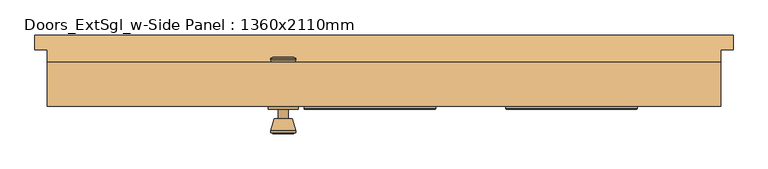
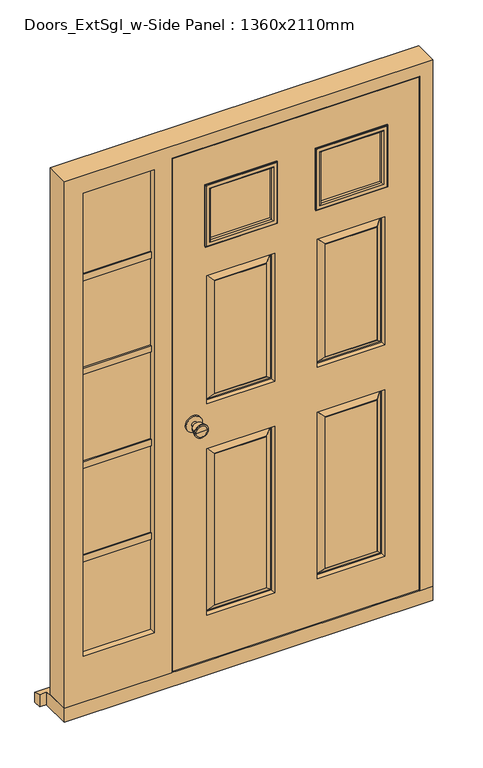
"""IFC4 building model written with IfcOpenShell, lengths in millimetres: door geometry, Doors_ExtSgl_w-Side Panel : 1360x2110mm."""

from ifc_helpers import new_model, si_unit, point, frame, frame_2d, origin, place, context, project, spatial, polyline, circle_curve, ellipse_curve, trimmed, segment, composite_curve, outline, extrude, faceted_brep, source, transform, mapped, element, save
from ifc_brep_helpers import plane_surface, cylinder_surface, revolved_surface, advanced_brep


def doors_extsgl_w_side_panel_1360x2110mm_f8072bf0(model_context):
    return source(origin(), model_context, "Body", "SolidModel", [
        advanced_brep(
        [(-352.5, 25.0, 1000.0), (-342.5, 25.0, 1000.0), (-362.5, 25.0, 1000.0), (-332.0241324, -24.0, 1000.0), (-352.5, -24.0, 1000.0), (-372.9758676, -24.0, 1000.0), (-327.5, -22.1721319, 1000.0), (-377.5, -22.1721319, 1000.0), (-327.5, -18.7084537, 1000.0), (-377.5, -18.7084537, 1000.0), (-333.863764, 6.0, 1000.0), (-371.136236, 6.0, 1000.0), (-342.5, 6.0, 1000.0), (-362.5, 6.0, 1000.0)],
        [
            (0, 1),
            (1, 2, circle_curve(frame((-352.5, 25.0, 1000.0), z_axis=(0.0, 1.0, 0.0), x_axis=(-1.0, 0.0, 0.0)), 10.0)),
            (2, 0),
            (2, 1, circle_curve(frame((-352.5, 25.0, 1000.0), z_axis=(0.0, 1.0, 0.0), x_axis=(-1.0, 0.0, 0.0)), 10.0)),
            (3, 4),
            (4, 5),
            (5, 3, circle_curve(frame((-352.5, -24.0, 1000.0), z_axis=(0.0, -1.0, 0.0), x_axis=(-1.0, 0.0, 0.0)), 20.4758676)),
            (3, 5, circle_curve(frame((-352.5, -24.0, 1000.0), z_axis=(0.0, -1.0, 0.0), x_axis=(-1.0, 0.0, 0.0)), 20.4758676)),
            (6, 3),
            (5, 7),
            (7, 6, circle_curve(frame((-352.5, -22.1721319, 1000.0), z_axis=(0.0, -1.0, 0.0), x_axis=(-1.0, 0.0, 0.0)), 25.0)),
            (6, 7, circle_curve(frame((-352.5, -22.1721319, 1000.0), z_axis=(0.0, -1.0, 0.0), x_axis=(-1.0, 0.0, 0.0)), 25.0)),
            (8, 6),
            (7, 9),
            (9, 8, circle_curve(frame((-352.5, -18.7084537, 1000.0), z_axis=(0.0, -1.0, 0.0), x_axis=(-1.0, 0.0, 0.0)), 25.0)),
            (8, 9, circle_curve(frame((-352.5, -18.7084537, 1000.0), z_axis=(0.0, -1.0, 0.0), x_axis=(-1.0, 0.0, 0.0)), 25.0)),
            (10, 8),
            (9, 11),
            (11, 10, circle_curve(frame((-352.5, 6.0, 1000.0), z_axis=(0.0, -1.0, 0.0), x_axis=(-1.0, 0.0, 0.0)), 18.636236)),
            (10, 11, circle_curve(frame((-352.5, 6.0, 1000.0), z_axis=(0.0, -1.0, 0.0), x_axis=(-1.0, 0.0, 0.0)), 18.636236)),
            (12, 10),
            (11, 13),
            (13, 12, circle_curve(frame((-352.5, 6.0, 1000.0), z_axis=(0.0, -1.0, 0.0), x_axis=(-1.0, 0.0, 0.0)), 10.0)),
            (12, 13, circle_curve(frame((-352.5, 6.0, 1000.0), z_axis=(0.0, -1.0, 0.0), x_axis=(-1.0, 0.0, 0.0)), 10.0)),
            (1, 12),
            (13, 2),
        ],
        [
            plane_surface(frame((-352.5, 25.0, 1000.0), z_axis=(0.0, 1.0, 0.0), x_axis=(-1.0, 0.0, 0.0))),
            plane_surface(frame((-352.5, -24.0, 1000.0), z_axis=(0.0, -1.0, 0.0), x_axis=(-1.0, 0.0, 0.0))),
            revolved_surface(polyline([(-372.9758676, -24.0, 1000.0), (-377.5, -22.1721319, 1000.0)]), (-352.5, 25.0, 1000.0), (0.0, 1.0, 0.0)),
            cylinder_surface(frame((-352.5, 25.0, 1000.0), z_axis=(0.0, 1.0, 0.0), x_axis=(-1.0, 0.0, 0.0)), 25.0),
            revolved_surface(polyline([(-377.5, -18.7084537, 1000.0), (-371.136236, 6.0, 1000.0)]), (-352.5, 25.0, 1000.0), (0.0, 1.0, 0.0)),
            plane_surface(frame((-352.5, 6.0, 1000.0), z_axis=(0.0, 1.0, 0.0), x_axis=(-1.0, 0.0, 0.0))),
            cylinder_surface(frame((-352.5, 25.0, 1000.0), z_axis=(0.0, 1.0, 0.0), x_axis=(-1.0, 0.0, 0.0)), 10.0),
        ],
        [
            (0, [[1, 2, 3]]),
            (0, [[-3, 4, -1]]),
            (1, [[5, 6, 7]]),
            (1, [[-6, -5, 8]]),
            (2, [[9, -7, 10, 11]]),
            (2, [[-10, -8, -9, 12]]),
            (3, [[13, -11, 14, 15]]),
            (3, [[-14, -12, -13, 16]]),
            (4, [[17, -15, 18, 19]]),
            (4, [[-18, -16, -17, 20]]),
            (5, [[21, -19, 22, 23]]),
            (5, [[-22, -20, -21, 24]]),
            (6, [[25, -23, 26, -2]]),
            (6, [[-26, -24, -25, -4]]),
        ],
    ),
        extrude(outline(composite_curve([segment(trimmed(circle_curve(frame_2d((1000.0, -352.5)), 30.0), [point((1000.0, -382.5))], [point((1000.0, -322.5))], False, "CARTESIAN"), True, "CONTINUOUS"), segment(trimmed(circle_curve(frame_2d((1000.0, -352.5)), 30.0), [point((1000.0, -322.5))], [point((1000.0, -382.5))], False, "CARTESIAN"), True, "CONTINUOUS")], self_intersect=False)), frame((0.0, 25.0, 0.0), z_axis=(0.0, 1.0, 0.0), x_axis=(0.0, 0.0, 1.0)), (0.0, 0.0, 1.0), 6.0),
        advanced_brep(
        [(-352.5, 81.0, 1000.0), (-362.5, 81.0, 1000.0), (-342.5, 81.0, 1000.0), (-332.0241324, 130.0, 1000.0), (-372.9758676, 130.0, 1000.0), (-352.5, 130.0, 1000.0), (-327.5, 128.1721319, 1000.0), (-377.5, 128.1721319, 1000.0), (-327.5, 124.7084537, 1000.0), (-377.5, 124.7084537, 1000.0), (-333.863764, 100.0, 1000.0), (-371.136236, 100.0, 1000.0), (-342.5, 100.0, 1000.0), (-362.5, 100.0, 1000.0)],
        [
            (0, 1),
            (1, 2, circle_curve(frame((-352.5, 81.0, 1000.0), z_axis=(0.0, -1.0, 0.0), x_axis=(-1.0, 0.0, 0.0)), 10.0)),
            (2, 0),
            (2, 1, circle_curve(frame((-352.5, 81.0, 1000.0), z_axis=(0.0, -1.0, 0.0), x_axis=(-1.0, 0.0, 0.0)), 10.0)),
            (3, 4, circle_curve(frame((-352.5, 130.0, 1000.0), z_axis=(0.0, 1.0, 0.0), x_axis=(-1.0, 0.0, 0.0)), 20.4758676)),
            (4, 5),
            (5, 3),
            (4, 3, circle_curve(frame((-352.5, 130.0, 1000.0), z_axis=(0.0, 1.0, 0.0), x_axis=(-1.0, 0.0, 0.0)), 20.4758676)),
            (6, 7, circle_curve(frame((-352.5, 128.1721319, 1000.0), z_axis=(0.0, 1.0, 0.0), x_axis=(-1.0, 0.0, 0.0)), 25.0)),
            (7, 4),
            (3, 6),
            (7, 6, circle_curve(frame((-352.5, 128.1721319, 1000.0), z_axis=(0.0, 1.0, 0.0), x_axis=(-1.0, 0.0, 0.0)), 25.0)),
            (8, 9, circle_curve(frame((-352.5, 124.7084537, 1000.0), z_axis=(0.0, 1.0, 0.0), x_axis=(-1.0, 0.0, 0.0)), 25.0)),
            (9, 7),
            (6, 8),
            (9, 8, circle_curve(frame((-352.5, 124.7084537, 1000.0), z_axis=(0.0, 1.0, 0.0), x_axis=(-1.0, 0.0, 0.0)), 25.0)),
            (10, 11, circle_curve(frame((-352.5, 100.0, 1000.0), z_axis=(0.0, 1.0, 0.0), x_axis=(-1.0, 0.0, 0.0)), 18.636236)),
            (11, 9),
            (8, 10),
            (11, 10, circle_curve(frame((-352.5, 100.0, 1000.0), z_axis=(0.0, 1.0, 0.0), x_axis=(-1.0, 0.0, 0.0)), 18.636236)),
            (12, 13, circle_curve(frame((-352.5, 100.0, 1000.0), z_axis=(0.0, 1.0, 0.0), x_axis=(-1.0, 0.0, 0.0)), 10.0)),
            (13, 11),
            (10, 12),
            (13, 12, circle_curve(frame((-352.5, 100.0, 1000.0), z_axis=(0.0, 1.0, 0.0), x_axis=(-1.0, 0.0, 0.0)), 10.0)),
            (1, 13),
            (12, 2),
        ],
        [
            plane_surface(frame((-352.5, 81.0, 1000.0), z_axis=(0.0, -1.0, 0.0), x_axis=(-1.0, 0.0, 0.0))),
            plane_surface(frame((-352.5, 130.0, 1000.0), z_axis=(0.0, 1.0, 0.0), x_axis=(-1.0, 0.0, 0.0))),
            revolved_surface(polyline([(-372.9758676, 130.0, 1000.0), (-377.5, 128.1721319, 1000.0)]), (-352.5, 81.0, 1000.0), (0.0, -1.0, 0.0)),
            cylinder_surface(frame((-352.5, 81.0, 1000.0), z_axis=(0.0, -1.0, 0.0), x_axis=(-1.0, 0.0, 0.0)), 25.0),
            revolved_surface(polyline([(-377.5, 124.7084537, 1000.0), (-371.136236, 100.0, 1000.0)]), (-352.5, 81.0, 1000.0), (0.0, -1.0, 0.0)),
            plane_surface(frame((-352.5, 100.0, 1000.0), z_axis=(0.0, -1.0, 0.0), x_axis=(-1.0, 0.0, 0.0))),
            cylinder_surface(frame((-352.5, 81.0, 1000.0), z_axis=(0.0, -1.0, 0.0), x_axis=(-1.0, 0.0, 0.0)), 10.0),
        ],
        [
            (0, [[1, 2, 3]]),
            (0, [[-3, 4, -1]]),
            (1, [[5, 6, 7]]),
            (1, [[8, -7, -6]]),
            (2, [[9, 10, -5, 11]]),
            (2, [[12, -11, -8, -10]]),
            (3, [[13, 14, -9, 15]]),
            (3, [[16, -15, -12, -14]]),
            (4, [[17, 18, -13, 19]]),
            (4, [[20, -19, -16, -18]]),
            (5, [[21, 22, -17, 23]]),
            (5, [[24, -23, -20, -22]]),
            (6, [[-2, 25, -21, 26]]),
            (6, [[-4, -26, -24, -25]]),
        ],
    ),
        extrude(outline(composite_curve([segment(trimmed(circle_curve(frame_2d((1000.0, -352.5)), 30.0), [point((1000.0, -382.5))], [point((1000.0, -322.5))], False, "CARTESIAN"), True, "CONTINUOUS"), segment(trimmed(circle_curve(frame_2d((1000.0, -352.5)), 30.0), [point((1000.0, -322.5))], [point((1000.0, -382.5))], False, "CARTESIAN"), True, "CONTINUOUS")], self_intersect=False)), frame((0.0, 75.0, 0.0), z_axis=(0.0, 1.0, 0.0), x_axis=(0.0, 0.0, 1.0)), (0.0, 0.0, 1.0), 6.0),
        faceted_brep([(460.5, 120.0, 54.5), (531.0, 120.0, 54.5), (531.0, 31.0, 54.5), (482.5, 31.0, 54.5), (482.5, 78.0, 54.5), (460.5, 78.0, 54.5), (460.5, 120.0, 2039.5), (-410.5, 120.0, 2039.5), (-410.5, 120.0, 54.5), (-829.0, 120.0, 54.5), (-829.0, 120.0, 2110.0), (531.0, 120.0, 2110.0), (-496.5, 120.0, 2039.5), (-758.5, 120.0, 2039.5), (-758.5, 120.0, 233.5), (-496.5, 120.0, 233.5), (531.0, 31.0, 2110.0), (-829.0, 31.0, 2110.0), (-829.0, 31.0, 54.5), (-432.5, 31.0, 54.5), (-432.5, 31.0, 2061.5), (482.5, 31.0, 2061.5), (-496.5, 31.0, 233.5), (-758.5, 31.0, 233.5), (-758.5, 31.0, 2039.5), (-496.5, 31.0, 2039.5), (482.5, 78.0, 2061.5), (-432.5, 78.0, 2061.5), (-432.5, 78.0, 54.5), (-410.5, 78.0, 54.5), (-410.5, 78.0, 2039.5), (460.5, 78.0, 2039.5), (-474.5, 78.0, 2061.5), (-780.5, 78.0, 2061.5), (-780.5, 78.0, 218.5), (-474.5, 78.0, 218.5), (-758.5, 78.0, 2039.5), (-496.5, 78.0, 2039.5), (-496.5, 78.0, 233.5), (-758.5, 78.0, 233.5), (-496.5, 54.0, 233.5), (-758.5, 54.0, 233.5), (-758.5, 54.0, 2039.5), (-496.5, 54.0, 2039.5), (-780.5, 54.0, 2061.5), (-780.5, 54.0, 218.5), (-474.5, 54.0, 218.5), (-474.5, 54.0, 2061.5)], [[[0, 1, 2, 3, 4, 5]], [[1, 0, 6, 7, 8, 9, 10, 11], [12, 13, 14, 15]], [[2, 1, 11, 16]], [[3, 2, 16, 17, 18, 19, 20, 21], [22, 23, 24, 25]], [[4, 3, 21, 26]], [[5, 4, 26, 27, 28, 29, 30, 31]], [[32, 33, 34, 35], [36, 37, 38, 39]], [[0, 5, 31, 6]], [[29, 8, 7, 30]], [[18, 9, 8, 29, 28, 19]], [[10, 9, 18, 17]], [[13, 36, 39, 14]], [[39, 38, 15, 14]], [[37, 12, 15, 38]], [[23, 22, 40, 41]], [[24, 23, 41, 42]], [[22, 25, 43, 40]], [[19, 28, 27, 20]], [[44, 45, 34, 33]], [[45, 46, 35, 34]], [[46, 47, 32, 35]], [[46, 45, 44, 47], [41, 40, 43, 42]], [[11, 10, 17, 16]], [[26, 21, 20, 27]], [[33, 32, 47, 44]], [[6, 31, 30, 7]], [[36, 13, 12, 37]], [[25, 24, 42, 43]]]),
        extrude(outline(polyline([(354.5, 41.0), (104.5, 41.0), (104.5, 65.0), (354.5, 65.0), (354.5, 41.0)])), frame((0.0, 0.0, 1683.5), z_axis=(0.0, 0.0, 1.0), x_axis=(1.0, 0.0, 0.0)), (0.0, 0.0, 1.0), 225.0),
        extrude(outline(polyline([(-52.5, 41.0), (-302.5, 41.0), (-302.5, 65.0), (-52.5, 65.0), (-52.5, 41.0)])), frame((0.0, 0.0, 1683.5), z_axis=(0.0, 0.0, 1.0), x_axis=(1.0, 0.0, 0.0)), (0.0, 0.0, 1.0), 225.0),
        faceted_brep([(556.0, 175.0, 0.0), (556.0, 175.0, 38.5947221), (556.0, 145.0, 47.2703282), (556.0, 145.0, 0.0), (-854.0, 175.0, 38.5947221), (-854.0, 175.0, 0.0), (-854.0, 145.0, 0.0), (-854.0, 145.0, 47.2703282), (531.0, 145.0, 0.0), (531.0, 31.0, 0.0), (-829.0, 31.0, 0.0), (-829.0, 145.0, 0.0), (-829.0, 145.0, 47.2703282), (-829.0, 120.0, 54.5), (531.0, 120.0, 54.5), (531.0, 145.0, 47.2703282), (-829.0, 31.0, 54.5), (531.0, 31.0, 54.5)], [[[0, 1, 2, 3]], [[4, 5, 6, 7]], [[5, 0, 3, 8, 9, 10, 11, 6]], [[1, 0, 5, 4]], [[1, 4, 7, 12, 13, 14, 15, 2]], [[13, 16, 17, 14]], [[16, 10, 9, 17]], [[12, 11, 10, 16, 13]], [[11, 12, 7, 6]], [[8, 15, 14, 17, 9]], [[15, 8, 3, 2]]]),
        faceted_brep([(479.5, 31.0, 58.5), (479.5, 31.0, 2058.5), (-427.5, 31.0, 2058.5), (-427.5, 31.0, 58.5), (104.5, 31.0, 1683.5), (104.5, 31.0, 1908.5), (354.5, 31.0, 1908.5), (354.5, 31.0, 1683.5), (-302.5, 31.0, 1683.5), (-302.5, 31.0, 1908.5), (-52.5, 31.0, 1908.5), (-52.5, 31.0, 1683.5), (-52.5, 31.0, 883.5), (-52.5, 31.0, 233.5), (-302.5, 31.0, 233.5), (-302.5, 31.0, 883.5), (354.5, 31.0, 883.5), (354.5, 31.0, 233.5), (104.5, 31.0, 233.5), (104.5, 31.0, 883.5), (-52.5, 31.0, 1558.5), (-52.5, 31.0, 1058.5), (-302.5, 31.0, 1058.5), (-302.5, 31.0, 1558.5), (354.5, 31.0, 1558.5), (354.5, 31.0, 1058.5), (104.5, 31.0, 1058.5), (104.5, 31.0, 1558.5), (-82.5, 31.0, 263.5), (-82.5, 31.0, 853.5), (-272.5, 31.0, 853.5), (-272.5, 31.0, 263.5), (324.5, 31.0, 263.5), (324.5, 31.0, 853.5), (134.5, 31.0, 853.5), (134.5, 31.0, 263.5), (-82.5, 31.0, 1088.5), (-82.5, 31.0, 1528.5), (-272.5, 31.0, 1528.5), (-272.5, 31.0, 1088.5), (324.5, 31.0, 1088.5), (324.5, 31.0, 1528.5), (134.5, 31.0, 1528.5), (134.5, 31.0, 1088.5), (479.5, 75.0, 58.5), (-427.5, 75.0, 58.5), (-427.5, 75.0, 2058.5), (479.5, 75.0, 2058.5), (104.5, 75.0, 1683.5), (354.5, 75.0, 1683.5), (354.5, 75.0, 1908.5), (104.5, 75.0, 1908.5), (-302.5, 75.0, 1683.5), (-52.5, 75.0, 1683.5), (-52.5, 75.0, 1908.5), (-302.5, 75.0, 1908.5), (104.5, 75.0, 883.5), (104.5, 75.0, 233.5), (354.5, 75.0, 233.5), (354.5, 75.0, 883.5), (-302.5, 75.0, 883.5), (-302.5, 75.0, 233.5), (-52.5, 75.0, 233.5), (-52.5, 75.0, 883.5), (104.5, 75.0, 1558.5), (104.5, 75.0, 1058.5), (354.5, 75.0, 1058.5), (354.5, 75.0, 1558.5), (-302.5, 75.0, 1558.5), (-302.5, 75.0, 1058.5), (-52.5, 75.0, 1058.5), (-52.5, 75.0, 1558.5), (134.5, 75.0, 263.5), (134.5, 75.0, 853.5), (324.5, 75.0, 853.5), (324.5, 75.0, 263.5), (-272.5, 75.0, 263.5), (-272.5, 75.0, 853.5), (-82.5, 75.0, 853.5), (-82.5, 75.0, 263.5), (134.5, 75.0, 1088.5), (134.5, 75.0, 1528.5), (324.5, 75.0, 1528.5), (324.5, 75.0, 1088.5), (-272.5, 75.0, 1088.5), (-272.5, 75.0, 1528.5), (-82.5, 75.0, 1528.5), (-82.5, 75.0, 1088.5), (107.5, 60.0, 880.5), (107.5, 60.0, 236.5), (132.5, 74.0, 855.5), (132.5, 74.0, 261.5), (112.5, 60.0, 241.5), (112.5, 60.0, 875.5), (134.5, 74.0, 263.5), (134.5, 74.0, 853.5), (351.5, 60.0, 236.5), (326.5, 74.0, 261.5), (346.5, 60.0, 241.5), (324.5, 74.0, 263.5), (351.5, 60.0, 880.5), (326.5, 74.0, 855.5), (346.5, 60.0, 875.5), (324.5, 74.0, 853.5), (-299.5, 60.0, 880.5), (-299.5, 60.0, 236.5), (-274.5, 74.0, 855.5), (-274.5, 74.0, 261.5), (-294.5, 60.0, 241.5), (-294.5, 60.0, 875.5), (-272.5, 74.0, 263.5), (-272.5, 74.0, 853.5), (-55.5, 60.0, 236.5), (-80.5, 74.0, 261.5), (-60.5, 60.0, 241.5), (-82.5, 74.0, 263.5), (-55.5, 60.0, 880.5), (-80.5, 74.0, 855.5), (-60.5, 60.0, 875.5), (-82.5, 74.0, 853.5), (-82.5, 32.0, 263.5), (-82.5, 32.0, 853.5), (-60.5, 46.0, 241.5), (-60.5, 46.0, 875.5), (-80.5, 32.0, 855.5), (-80.5, 32.0, 261.5), (-55.5, 46.0, 880.5), (-55.5, 46.0, 236.5), (-272.5, 32.0, 853.5), (-294.5, 46.0, 875.5), (-274.5, 32.0, 855.5), (-299.5, 46.0, 880.5), (-272.5, 32.0, 263.5), (-294.5, 46.0, 241.5), (-274.5, 32.0, 261.5), (-299.5, 46.0, 236.5), (351.5, 46.0, 880.5), (351.5, 46.0, 236.5), (326.5, 32.0, 855.5), (326.5, 32.0, 261.5), (346.5, 46.0, 241.5), (346.5, 46.0, 875.5), (324.5, 32.0, 263.5), (324.5, 32.0, 853.5), (107.5, 46.0, 236.5), (132.5, 32.0, 261.5), (112.5, 46.0, 241.5), (134.5, 32.0, 263.5), (107.5, 46.0, 880.5), (132.5, 32.0, 855.5), (112.5, 46.0, 875.5), (134.5, 32.0, 853.5), (134.5, 74.0, 1088.5), (134.5, 74.0, 1528.5), (112.5, 60.0, 1066.5), (112.5, 60.0, 1550.5), (132.5, 74.0, 1530.5), (132.5, 74.0, 1086.5), (107.5, 60.0, 1555.5), (107.5, 60.0, 1061.5), (324.5, 74.0, 1528.5), (346.5, 60.0, 1550.5), (326.5, 74.0, 1530.5), (351.5, 60.0, 1555.5), (324.5, 74.0, 1088.5), (346.5, 60.0, 1066.5), (326.5, 74.0, 1086.5), (351.5, 60.0, 1061.5), (-272.5, 74.0, 1088.5), (-272.5, 74.0, 1528.5), (-294.5, 60.0, 1066.5), (-294.5, 60.0, 1550.5), (-274.5, 74.0, 1530.5), (-274.5, 74.0, 1086.5), (-299.5, 60.0, 1555.5), (-299.5, 60.0, 1061.5), (-82.5, 74.0, 1528.5), (-60.5, 60.0, 1550.5), (-80.5, 74.0, 1530.5), (-55.5, 60.0, 1555.5), (-82.5, 74.0, 1088.5), (-60.5, 60.0, 1066.5), (-80.5, 74.0, 1086.5), (-55.5, 60.0, 1061.5), (-82.5, 32.0, 1088.5), (-82.5, 32.0, 1528.5), (-60.5, 46.0, 1066.5), (-60.5, 46.0, 1550.5), (-80.5, 32.0, 1530.5), (-80.5, 32.0, 1086.5), (-55.5, 46.0, 1555.5), (-55.5, 46.0, 1061.5), (-272.5, 32.0, 1528.5), (-294.5, 46.0, 1550.5), (-274.5, 32.0, 1530.5), (-299.5, 46.0, 1555.5), (-272.5, 32.0, 1088.5), (-294.5, 46.0, 1066.5), (-274.5, 32.0, 1086.5), (-299.5, 46.0, 1061.5), (351.5, 46.0, 1555.5), (351.5, 46.0, 1061.5), (326.5, 32.0, 1530.5), (326.5, 32.0, 1086.5), (346.5, 46.0, 1066.5), (346.5, 46.0, 1550.5), (324.5, 32.0, 1088.5), (324.5, 32.0, 1528.5), (107.5, 46.0, 1061.5), (132.5, 32.0, 1086.5), (112.5, 46.0, 1066.5), (134.5, 32.0, 1088.5), (107.5, 46.0, 1555.5), (132.5, 32.0, 1530.5), (112.5, 46.0, 1550.5), (134.5, 32.0, 1528.5)], [[[0, 1, 2, 3], [4, 5, 6, 7], [8, 9, 10, 11], [12, 13, 14, 15], [16, 17, 18, 19], [20, 21, 22, 23], [24, 25, 26, 27]], [[28, 29, 30, 31]], [[32, 33, 34, 35]], [[36, 37, 38, 39]], [[40, 41, 42, 43]], [[44, 45, 46, 47], [48, 49, 50, 51], [52, 53, 54, 55], [56, 57, 58, 59], [60, 61, 62, 63], [64, 65, 66, 67], [68, 69, 70, 71]], [[72, 73, 74, 75]], [[76, 77, 78, 79]], [[80, 81, 82, 83]], [[84, 85, 86, 87]], [[1, 0, 44, 47]], [[2, 1, 47, 46]], [[3, 2, 46, 45]], [[0, 3, 45, 44]], [[5, 4, 48, 51]], [[6, 5, 51, 50]], [[7, 6, 50, 49]], [[4, 7, 49, 48]], [[9, 8, 52, 55]], [[10, 9, 55, 54]], [[11, 10, 54, 53]], [[8, 11, 53, 52]], [[88, 89, 57, 56]], [[90, 91, 92, 93]], [[72, 94, 95, 73]], [[57, 89, 96, 58]], [[92, 91, 97, 98]], [[94, 72, 75, 99]], [[58, 96, 100, 59]], [[98, 97, 101, 102]], [[99, 75, 74, 103]], [[88, 56, 59, 100]], [[89, 88, 100, 96], [93, 92, 98, 102]], [[90, 93, 102, 101]], [[91, 90, 101, 97], [95, 94, 99, 103]], [[73, 95, 103, 74]], [[104, 105, 61, 60]], [[106, 107, 108, 109]], [[76, 110, 111, 77]], [[61, 105, 112, 62]], [[108, 107, 113, 114]], [[110, 76, 79, 115]], [[62, 112, 116, 63]], [[114, 113, 117, 118]], [[115, 79, 78, 119]], [[104, 60, 63, 116]], [[105, 104, 116, 112], [109, 108, 114, 118]], [[106, 109, 118, 117]], [[107, 106, 117, 113], [111, 110, 115, 119]], [[77, 111, 119, 78]], [[120, 121, 29, 28]], [[122, 123, 124, 125]], [[12, 126, 127, 13]], [[29, 121, 128, 30]], [[124, 123, 129, 130]], [[126, 12, 15, 131]], [[30, 128, 132, 31]], [[130, 129, 133, 134]], [[131, 15, 14, 135]], [[120, 28, 31, 132]], [[125, 124, 130, 134], [121, 120, 132, 128]], [[122, 125, 134, 133]], [[127, 126, 131, 135], [123, 122, 133, 129]], [[13, 127, 135, 14]], [[136, 137, 17, 16]], [[138, 139, 140, 141]], [[32, 142, 143, 33]], [[17, 137, 144, 18]], [[140, 139, 145, 146]], [[142, 32, 35, 147]], [[18, 144, 148, 19]], [[146, 145, 149, 150]], [[147, 35, 34, 151]], [[136, 16, 19, 148]], [[137, 136, 148, 144], [141, 140, 146, 150]], [[138, 141, 150, 149]], [[139, 138, 149, 145], [143, 142, 147, 151]], [[33, 143, 151, 34]], [[152, 153, 81, 80]], [[154, 155, 156, 157]], [[64, 158, 159, 65]], [[81, 153, 160, 82]], [[156, 155, 161, 162]], [[158, 64, 67, 163]], [[82, 160, 164, 83]], [[162, 161, 165, 166]], [[163, 67, 66, 167]], [[152, 80, 83, 164]], [[157, 156, 162, 166], [153, 152, 164, 160]], [[154, 157, 166, 165]], [[159, 158, 163, 167], [155, 154, 165, 161]], [[65, 159, 167, 66]], [[168, 169, 85, 84]], [[170, 171, 172, 173]], [[68, 174, 175, 69]], [[85, 169, 176, 86]], [[172, 171, 177, 178]], [[174, 68, 71, 179]], [[86, 176, 180, 87]], [[178, 177, 181, 182]], [[179, 71, 70, 183]], [[168, 84, 87, 180]], [[173, 172, 178, 182], [169, 168, 180, 176]], [[170, 173, 182, 181]], [[175, 174, 179, 183], [171, 170, 181, 177]], [[69, 175, 183, 70]], [[184, 185, 37, 36]], [[186, 187, 188, 189]], [[20, 190, 191, 21]], [[37, 185, 192, 38]], [[188, 187, 193, 194]], [[190, 20, 23, 195]], [[38, 192, 196, 39]], [[194, 193, 197, 198]], [[195, 23, 22, 199]], [[184, 36, 39, 196]], [[189, 188, 194, 198], [185, 184, 196, 192]], [[186, 189, 198, 197]], [[191, 190, 195, 199], [187, 186, 197, 193]], [[21, 191, 199, 22]], [[200, 201, 25, 24]], [[202, 203, 204, 205]], [[40, 206, 207, 41]], [[25, 201, 208, 26]], [[204, 203, 209, 210]], [[206, 40, 43, 211]], [[26, 208, 212, 27]], [[210, 209, 213, 214]], [[211, 43, 42, 215]], [[200, 24, 27, 212]], [[201, 200, 212, 208], [205, 204, 210, 214]], [[202, 205, 214, 213]], [[203, 202, 213, 209], [207, 206, 211, 215]], [[41, 207, 215, 42]]]),
        advanced_brep(
        [(362.5, 27.0, 1675.5), (362.5, 31.0, 1675.5), (362.5, 31.0, 1916.5), (362.5, 27.0, 1916.5), (360.5, 25.0, 1677.5), (360.5, 25.0, 1914.5), (342.5, 30.0, 1695.5), (347.5, 25.0, 1690.5), (347.5, 25.0, 1901.5), (342.5, 30.0, 1896.5), (342.5, 41.0, 1695.5), (342.5, 41.0, 1896.5), (354.5, 31.0, 1683.5), (354.5, 41.0, 1683.5), (354.5, 41.0, 1908.5), (354.5, 31.0, 1908.5), (96.5, 31.0, 1916.5), (96.5, 27.0, 1916.5), (98.5, 25.0, 1914.5), (111.5, 25.0, 1901.5), (116.5, 30.0, 1896.5), (116.5, 41.0, 1896.5), (104.5, 41.0, 1908.5), (104.5, 31.0, 1908.5), (96.5, 31.0, 1675.5), (96.5, 27.0, 1675.5), (98.5, 25.0, 1677.5), (111.5, 25.0, 1690.5), (116.5, 30.0, 1695.5), (116.5, 41.0, 1695.5), (104.5, 41.0, 1683.5), (104.5, 31.0, 1683.5)],
        [
            (0, 1),
            (1, 2),
            (2, 3),
            (3, 0),
            (4, 0, ellipse_curve(frame((360.5, 27.0, 1677.5), z_axis=(0.7071067811865475, 0.0, 0.7071067811865475), x_axis=(0.7071067811865474, 0.0, -0.7071067811865476)), 2.8284271, 2.0)),
            (3, 5, ellipse_curve(frame((360.5, 27.0, 1914.5), z_axis=(0.7071067811865475, 0.0, -0.7071067811865475), x_axis=(-0.7071067811865474, 0.0, -0.7071067811865476)), 2.8284271, 2.0)),
            (5, 4),
            (6, 7, ellipse_curve(frame((347.5, 30.0, 1690.5), z_axis=(0.7071067811865475, 0.0, 0.7071067811865475), x_axis=(0.7071067811865474, 0.0, -0.7071067811865476)), 7.0710678, 5.0)),
            (7, 8),
            (8, 9, ellipse_curve(frame((347.5, 30.0, 1901.5), z_axis=(0.7071067811865475, 0.0, -0.7071067811865475), x_axis=(-0.7071067811865474, 0.0, -0.7071067811865476)), 7.0710678, 5.0)),
            (9, 6),
            (10, 6),
            (9, 11),
            (11, 10),
            (12, 13),
            (13, 14),
            (14, 15),
            (15, 12),
            (2, 16),
            (16, 17),
            (17, 3),
            (17, 18, ellipse_curve(frame((98.5, 27.0, 1914.5), z_axis=(0.7071067811865475, 0.0, 0.7071067811865475), x_axis=(0.7071067811865476, 0.0, -0.7071067811865474)), 2.8284271, 2.0)),
            (18, 5),
            (8, 19),
            (19, 20, ellipse_curve(frame((111.5, 30.0, 1901.5), z_axis=(0.7071067811865475, 0.0, 0.7071067811865475), x_axis=(0.7071067811865476, 0.0, -0.7071067811865474)), 7.0710678, 5.0)),
            (20, 9),
            (20, 21),
            (21, 11),
            (14, 22),
            (22, 23),
            (23, 15),
            (16, 24),
            (24, 25),
            (25, 17),
            (25, 26, ellipse_curve(frame((98.5, 27.0, 1677.5), z_axis=(-0.7071067811865475, 0.0, 0.7071067811865475), x_axis=(0.7071067811865474, 0.0, 0.7071067811865476)), 2.8284271, 2.0)),
            (26, 18),
            (19, 27),
            (27, 28, ellipse_curve(frame((111.5, 30.0, 1690.5), z_axis=(-0.7071067811865475, 0.0, 0.7071067811865475), x_axis=(0.7071067811865474, 0.0, 0.7071067811865476)), 7.0710678, 5.0)),
            (28, 20),
            (28, 29),
            (29, 21),
            (22, 30),
            (30, 31),
            (31, 23),
            (24, 1),
            (0, 25),
            (4, 26),
            (7, 27),
            (6, 28),
            (10, 29),
            (13, 30),
            (12, 31),
        ],
        [
            plane_surface(frame((362.5, 31.0, 1675.5), z_axis=(1.0, 0.0, 0.0), x_axis=(0.0, 0.0, 1.0))),
            cylinder_surface(frame((360.5, 27.0, 1683.5), z_axis=(0.0, 0.0, -1.0), x_axis=(1.0, 0.0, 0.0)), 2.0),
            cylinder_surface(frame((347.5, 30.0, 1683.5), z_axis=(0.0, 0.0, -1.0), x_axis=(1.0, 0.0, 0.0)), 5.0),
            plane_surface(frame((342.5, 30.0, 1695.5), z_axis=(-1.0, 0.0, 0.0), x_axis=(0.0, 0.0, 1.0))),
            plane_surface(frame((354.5, 41.0, 1683.5), z_axis=(1.0, 0.0, 0.0), x_axis=(0.0, 0.0, 1.0))),
            plane_surface(frame((362.5, 31.0, 1916.5), z_axis=(0.0, 0.0, 1.0), x_axis=(-1.0, 0.0, 0.0))),
            cylinder_surface(frame((354.5, 27.0, 1914.5), z_axis=(1.0, 0.0, 0.0), x_axis=(0.0, 0.0, 1.0)), 2.0),
            cylinder_surface(frame((354.5, 30.0, 1901.5), z_axis=(1.0, 0.0, 0.0), x_axis=(0.0, 0.0, 1.0)), 5.0),
            plane_surface(frame((342.5, 30.0, 1896.5), z_axis=(0.0, 0.0, -1.0), x_axis=(-1.0, 0.0, 0.0))),
            plane_surface(frame((354.5, 41.0, 1908.5), z_axis=(0.0, 0.0, 1.0), x_axis=(-1.0, 0.0, 0.0))),
            plane_surface(frame((96.5, 31.0, 1916.5), z_axis=(-1.0, 0.0, 0.0), x_axis=(0.0, 0.0, -1.0))),
            cylinder_surface(frame((98.5, 27.0, 1908.5), z_axis=(0.0, 0.0, 1.0), x_axis=(-1.0, 0.0, 0.0)), 2.0),
            cylinder_surface(frame((111.5, 30.0, 1908.5), z_axis=(0.0, 0.0, 1.0), x_axis=(-1.0, 0.0, 0.0)), 5.0),
            plane_surface(frame((116.5, 30.0, 1896.5), z_axis=(1.0, 0.0, 0.0), x_axis=(0.0, 0.0, -1.0))),
            plane_surface(frame((104.5, 41.0, 1908.5), z_axis=(-1.0, 0.0, 0.0), x_axis=(0.0, 0.0, -1.0))),
            plane_surface(frame((96.5, 31.0, 1675.5), z_axis=(0.0, 0.0, -1.0), x_axis=(1.0, 0.0, 0.0))),
            cylinder_surface(frame((104.5, 27.0, 1677.5), z_axis=(-1.0, 0.0, 0.0), x_axis=(0.0, 0.0, -1.0)), 2.0),
            plane_surface(frame((98.5, 25.0, 1677.5), z_axis=(0.0, -1.0, 0.0), x_axis=(1.0, 0.0, 0.0))),
            cylinder_surface(frame((104.5, 30.0, 1690.5), z_axis=(-1.0, 0.0, 0.0), x_axis=(0.0, 0.0, -1.0)), 5.0),
            plane_surface(frame((116.5, 30.0, 1695.5), z_axis=(0.0, 0.0, 1.0), x_axis=(1.0, 0.0, 0.0))),
            plane_surface(frame((116.5, 41.0, 1695.5), z_axis=(0.0, 1.0, 0.0), x_axis=(1.0, 0.0, 0.0))),
            plane_surface(frame((104.5, 41.0, 1683.5), z_axis=(0.0, 0.0, -1.0), x_axis=(1.0, 0.0, 0.0))),
            plane_surface(frame((104.5, 31.0, 1683.5), z_axis=(0.0, 1.0, 0.0), x_axis=(1.0, 0.0, 0.0))),
        ],
        [
            (0, [[1, 2, 3, 4]]),
            (1, [[5, -4, 6, 7]]),
            (2, [[8, 9, 10, 11]]),
            (3, [[12, -11, 13, 14]]),
            (4, [[15, 16, 17, 18]]),
            (5, [[-3, 19, 20, 21]]),
            (6, [[-6, -21, 22, 23]]),
            (7, [[-10, 24, 25, 26]]),
            (8, [[-13, -26, 27, 28]]),
            (9, [[-17, 29, 30, 31]]),
            (10, [[-20, 32, 33, 34]]),
            (11, [[-22, -34, 35, 36]]),
            (12, [[-25, 37, 38, 39]]),
            (13, [[-27, -39, 40, 41]]),
            (14, [[-30, 42, 43, 44]]),
            (15, [[-33, 45, -1, 46]]),
            (16, [[-35, -46, -5, 47]]),
            (17, [[-23, -36, -47, -7], [48, -37, -24, -9]]),
            (18, [[-38, -48, -8, 49]]),
            (19, [[-40, -49, -12, 50]]),
            (20, [[51, -42, -29, -16], [-28, -41, -50, -14]]),
            (21, [[-43, -51, -15, 52]]),
            (22, [[-45, -32, -19, -2], [-31, -44, -52, -18]]),
        ],
    ),
        advanced_brep(
        [(-44.5, 27.0, 1675.5), (-44.5, 31.0, 1675.5), (-44.5, 31.0, 1916.5), (-44.5, 27.0, 1916.5), (-46.5, 25.0, 1677.5), (-46.5, 25.0, 1914.5), (-64.5, 30.0, 1695.5), (-59.5, 25.0, 1690.5), (-59.5, 25.0, 1901.5), (-64.5, 30.0, 1896.5), (-64.5, 41.0, 1695.5), (-64.5, 41.0, 1896.5), (-52.5, 31.0, 1683.5), (-52.5, 41.0, 1683.5), (-52.5, 41.0, 1908.5), (-52.5, 31.0, 1908.5), (-310.5, 31.0, 1916.5), (-310.5, 27.0, 1916.5), (-308.5, 25.0, 1914.5), (-295.5, 25.0, 1901.5), (-290.5, 30.0, 1896.5), (-290.5, 41.0, 1896.5), (-302.5, 41.0, 1908.5), (-302.5, 31.0, 1908.5), (-310.5, 31.0, 1675.5), (-310.5, 27.0, 1675.5), (-308.5, 25.0, 1677.5), (-295.5, 25.0, 1690.5), (-290.5, 30.0, 1695.5), (-290.5, 41.0, 1695.5), (-302.5, 41.0, 1683.5), (-302.5, 31.0, 1683.5)],
        [
            (0, 1),
            (1, 2),
            (2, 3),
            (3, 0),
            (4, 0, ellipse_curve(frame((-46.5, 27.0, 1677.5), z_axis=(0.7071067811865475, 0.0, 0.7071067811865475), x_axis=(0.7071067811865474, 0.0, -0.7071067811865476)), 2.8284271, 2.0)),
            (3, 5, ellipse_curve(frame((-46.5, 27.0, 1914.5), z_axis=(0.7071067811865475, 0.0, -0.7071067811865475), x_axis=(-0.7071067811865474, 0.0, -0.7071067811865476)), 2.8284271, 2.0)),
            (5, 4),
            (6, 7, ellipse_curve(frame((-59.5, 30.0, 1690.5), z_axis=(0.7071067811865475, 0.0, 0.7071067811865475), x_axis=(0.7071067811865474, 0.0, -0.7071067811865476)), 7.0710678, 5.0)),
            (7, 8),
            (8, 9, ellipse_curve(frame((-59.5, 30.0, 1901.5), z_axis=(0.7071067811865475, 0.0, -0.7071067811865475), x_axis=(-0.7071067811865474, 0.0, -0.7071067811865476)), 7.0710678, 5.0)),
            (9, 6),
            (10, 6),
            (9, 11),
            (11, 10),
            (12, 13),
            (13, 14),
            (14, 15),
            (15, 12),
            (2, 16),
            (16, 17),
            (17, 3),
            (17, 18, ellipse_curve(frame((-308.5, 27.0, 1914.5), z_axis=(0.7071067811865475, 0.0, 0.7071067811865475), x_axis=(0.7071067811865476, 0.0, -0.7071067811865474)), 2.8284271, 2.0)),
            (18, 5),
            (8, 19),
            (19, 20, ellipse_curve(frame((-295.5, 30.0, 1901.5), z_axis=(0.7071067811865475, 0.0, 0.7071067811865475), x_axis=(0.7071067811865476, 0.0, -0.7071067811865474)), 7.0710678, 5.0)),
            (20, 9),
            (20, 21),
            (21, 11),
            (14, 22),
            (22, 23),
            (23, 15),
            (16, 24),
            (24, 25),
            (25, 17),
            (25, 26, ellipse_curve(frame((-308.5, 27.0, 1677.5), z_axis=(-0.7071067811865475, 0.0, 0.7071067811865475), x_axis=(0.7071067811865474, 0.0, 0.7071067811865476)), 2.8284271, 2.0)),
            (26, 18),
            (19, 27),
            (27, 28, ellipse_curve(frame((-295.5, 30.0, 1690.5), z_axis=(-0.7071067811865475, 0.0, 0.7071067811865475), x_axis=(0.7071067811865474, 0.0, 0.7071067811865476)), 7.0710678, 5.0)),
            (28, 20),
            (28, 29),
            (29, 21),
            (22, 30),
            (30, 31),
            (31, 23),
            (24, 1),
            (0, 25),
            (4, 26),
            (7, 27),
            (6, 28),
            (10, 29),
            (13, 30),
            (12, 31),
        ],
        [
            plane_surface(frame((-44.5, 31.0, 1675.5), z_axis=(1.0, 0.0, 0.0), x_axis=(0.0, 0.0, 1.0))),
            cylinder_surface(frame((-46.5, 27.0, 1683.5), z_axis=(0.0, 0.0, -1.0), x_axis=(1.0, 0.0, 0.0)), 2.0),
            cylinder_surface(frame((-59.5, 30.0, 1683.5), z_axis=(0.0, 0.0, -1.0), x_axis=(1.0, 0.0, 0.0)), 5.0),
            plane_surface(frame((-64.5, 30.0, 1695.5), z_axis=(-1.0, 0.0, 0.0), x_axis=(0.0, 0.0, 1.0))),
            plane_surface(frame((-52.5, 41.0, 1683.5), z_axis=(1.0, 0.0, 0.0), x_axis=(0.0, 0.0, 1.0))),
            plane_surface(frame((-44.5, 31.0, 1916.5), z_axis=(0.0, 0.0, 1.0), x_axis=(-1.0, 0.0, 0.0))),
            cylinder_surface(frame((-52.5, 27.0, 1914.5), z_axis=(1.0, 0.0, 0.0), x_axis=(0.0, 0.0, 1.0)), 2.0),
            cylinder_surface(frame((-52.5, 30.0, 1901.5), z_axis=(1.0, 0.0, 0.0), x_axis=(0.0, 0.0, 1.0)), 5.0),
            plane_surface(frame((-64.5, 30.0, 1896.5), z_axis=(0.0, 0.0, -1.0), x_axis=(-1.0, 0.0, 0.0))),
            plane_surface(frame((-52.5, 41.0, 1908.5), z_axis=(0.0, 0.0, 1.0), x_axis=(-1.0, 0.0, 0.0))),
            plane_surface(frame((-310.5, 31.0, 1916.5), z_axis=(-1.0, 0.0, 0.0), x_axis=(0.0, 0.0, -1.0))),
            cylinder_surface(frame((-308.5, 27.0, 1908.5), z_axis=(0.0, 0.0, 1.0), x_axis=(-1.0, 0.0, 0.0)), 2.0),
            cylinder_surface(frame((-295.5, 30.0, 1908.5), z_axis=(0.0, 0.0, 1.0), x_axis=(-1.0, 0.0, 0.0)), 5.0),
            plane_surface(frame((-290.5, 30.0, 1896.5), z_axis=(1.0, 0.0, 0.0), x_axis=(0.0, 0.0, -1.0))),
            plane_surface(frame((-302.5, 41.0, 1908.5), z_axis=(-1.0, 0.0, 0.0), x_axis=(0.0, 0.0, -1.0))),
            plane_surface(frame((-310.5, 31.0, 1675.5), z_axis=(0.0, 0.0, -1.0), x_axis=(1.0, 0.0, 0.0))),
            cylinder_surface(frame((-302.5, 27.0, 1677.5), z_axis=(-1.0, 0.0, 0.0), x_axis=(0.0, 0.0, -1.0)), 2.0),
            plane_surface(frame((-308.5, 25.0, 1677.5), z_axis=(0.0, -1.0, 0.0), x_axis=(1.0, 0.0, 0.0))),
            cylinder_surface(frame((-302.5, 30.0, 1690.5), z_axis=(-1.0, 0.0, 0.0), x_axis=(0.0, 0.0, -1.0)), 5.0),
            plane_surface(frame((-290.5, 30.0, 1695.5), z_axis=(0.0, 0.0, 1.0), x_axis=(1.0, 0.0, 0.0))),
            plane_surface(frame((-290.5, 41.0, 1695.5), z_axis=(0.0, 1.0, 0.0), x_axis=(1.0, 0.0, 0.0))),
            plane_surface(frame((-302.5, 41.0, 1683.5), z_axis=(0.0, 0.0, -1.0), x_axis=(1.0, 0.0, 0.0))),
            plane_surface(frame((-302.5, 31.0, 1683.5), z_axis=(0.0, 1.0, 0.0), x_axis=(1.0, 0.0, 0.0))),
        ],
        [
            (0, [[1, 2, 3, 4]]),
            (1, [[5, -4, 6, 7]]),
            (2, [[8, 9, 10, 11]]),
            (3, [[12, -11, 13, 14]]),
            (4, [[15, 16, 17, 18]]),
            (5, [[-3, 19, 20, 21]]),
            (6, [[-6, -21, 22, 23]]),
            (7, [[-10, 24, 25, 26]]),
            (8, [[-13, -26, 27, 28]]),
            (9, [[-17, 29, 30, 31]]),
            (10, [[-20, 32, 33, 34]]),
            (11, [[-22, -34, 35, 36]]),
            (12, [[-25, 37, 38, 39]]),
            (13, [[-27, -39, 40, 41]]),
            (14, [[-30, 42, 43, 44]]),
            (15, [[-33, 45, -1, 46]]),
            (16, [[-35, -46, -5, 47]]),
            (17, [[-23, -36, -47, -7], [48, -37, -24, -9]]),
            (18, [[-38, -48, -8, 49]]),
            (19, [[-40, -49, -12, 50]]),
            (20, [[51, -42, -29, -16], [-28, -41, -50, -14]]),
            (21, [[-43, -51, -15, 52]]),
            (22, [[-45, -32, -19, -2], [-31, -44, -52, -18]]),
        ],
    ),
        advanced_brep(
        [(-310.5, 79.0, 1675.5), (-310.5, 75.0, 1675.5), (-310.5, 75.0, 1916.5), (-310.5, 79.0, 1916.5), (-308.5, 81.0, 1677.5), (-308.5, 81.0, 1914.5), (-290.5, 76.0, 1695.5), (-295.5, 81.0, 1690.5), (-295.5, 81.0, 1901.5), (-290.5, 76.0, 1896.5), (-290.5, 65.0, 1695.5), (-290.5, 65.0, 1896.5), (-302.5, 75.0, 1683.5), (-302.5, 65.0, 1683.5), (-302.5, 65.0, 1908.5), (-302.5, 75.0, 1908.5), (-44.5, 75.0, 1916.5), (-44.5, 79.0, 1916.5), (-46.5, 81.0, 1914.5), (-59.5, 81.0, 1901.5), (-64.5, 76.0, 1896.5), (-64.5, 65.0, 1896.5), (-52.5, 65.0, 1908.5), (-52.5, 75.0, 1908.5), (-44.5, 75.0, 1675.5), (-44.5, 79.0, 1675.5), (-46.5, 81.0, 1677.5), (-59.5, 81.0, 1690.5), (-64.5, 76.0, 1695.5), (-64.5, 65.0, 1695.5), (-52.5, 65.0, 1683.5), (-52.5, 75.0, 1683.5)],
        [
            (0, 1),
            (1, 2),
            (2, 3),
            (3, 0),
            (4, 0, ellipse_curve(frame((-308.5, 79.0, 1677.5), z_axis=(-0.7071067811865475, 0.0, 0.7071067811865475), x_axis=(-0.7071067811865474, 0.0, -0.7071067811865476)), 2.8284271, 2.0)),
            (3, 5, ellipse_curve(frame((-308.5, 79.0, 1914.5), z_axis=(-0.7071067811865475, 0.0, -0.7071067811865475), x_axis=(0.7071067811865474, 0.0, -0.7071067811865476)), 2.8284271, 2.0)),
            (5, 4),
            (6, 7, ellipse_curve(frame((-295.5, 76.0, 1690.5), z_axis=(-0.7071067811865475, 0.0, 0.7071067811865475), x_axis=(-0.7071067811865474, 0.0, -0.7071067811865476)), 7.0710678, 5.0)),
            (7, 8),
            (8, 9, ellipse_curve(frame((-295.5, 76.0, 1901.5), z_axis=(-0.7071067811865475, 0.0, -0.7071067811865475), x_axis=(0.7071067811865474, 0.0, -0.7071067811865476)), 7.0710678, 5.0)),
            (9, 6),
            (10, 6),
            (9, 11),
            (11, 10),
            (12, 13),
            (13, 14),
            (14, 15),
            (15, 12),
            (2, 16),
            (16, 17),
            (17, 3),
            (17, 18, ellipse_curve(frame((-46.5, 79.0, 1914.5), z_axis=(-0.7071067811865475, 0.0, 0.7071067811865475), x_axis=(-0.7071067811865476, 0.0, -0.7071067811865474)), 2.8284271, 2.0)),
            (18, 5),
            (8, 19),
            (19, 20, ellipse_curve(frame((-59.5, 76.0, 1901.5), z_axis=(-0.7071067811865475, 0.0, 0.7071067811865475), x_axis=(-0.7071067811865476, 0.0, -0.7071067811865474)), 7.0710678, 5.0)),
            (20, 9),
            (20, 21),
            (21, 11),
            (14, 22),
            (22, 23),
            (23, 15),
            (16, 24),
            (24, 25),
            (25, 17),
            (25, 26, ellipse_curve(frame((-46.5, 79.0, 1677.5), z_axis=(0.7071067811865475, 0.0, 0.7071067811865475), x_axis=(-0.7071067811865474, 0.0, 0.7071067811865476)), 2.8284271, 2.0)),
            (26, 18),
            (19, 27),
            (27, 28, ellipse_curve(frame((-59.5, 76.0, 1690.5), z_axis=(0.7071067811865475, 0.0, 0.7071067811865475), x_axis=(-0.7071067811865474, 0.0, 0.7071067811865476)), 7.0710678, 5.0)),
            (28, 20),
            (28, 29),
            (29, 21),
            (22, 30),
            (30, 31),
            (31, 23),
            (24, 1),
            (0, 25),
            (4, 26),
            (7, 27),
            (6, 28),
            (10, 29),
            (13, 30),
            (12, 31),
        ],
        [
            plane_surface(frame((-310.5, 75.0, 1675.5), z_axis=(-1.0, 0.0, 0.0), x_axis=(0.0, 0.0, 1.0))),
            cylinder_surface(frame((-308.5, 79.0, 1683.5), z_axis=(0.0, 0.0, -1.0), x_axis=(-1.0, 0.0, 0.0)), 2.0),
            cylinder_surface(frame((-295.5, 76.0, 1683.5), z_axis=(0.0, 0.0, -1.0), x_axis=(-1.0, 0.0, 0.0)), 5.0),
            plane_surface(frame((-290.5, 76.0, 1695.5), z_axis=(1.0, 0.0, 0.0), x_axis=(0.0, 0.0, 1.0))),
            plane_surface(frame((-302.5, 65.0, 1683.5), z_axis=(-1.0, 0.0, 0.0), x_axis=(0.0, 0.0, 1.0))),
            plane_surface(frame((-310.5, 75.0, 1916.5), z_axis=(0.0, 0.0, 1.0), x_axis=(1.0, 0.0, 0.0))),
            cylinder_surface(frame((-302.5, 79.0, 1914.5), z_axis=(-1.0, 0.0, 0.0), x_axis=(0.0, 0.0, 1.0)), 2.0),
            cylinder_surface(frame((-302.5, 76.0, 1901.5), z_axis=(-1.0, 0.0, 0.0), x_axis=(0.0, 0.0, 1.0)), 5.0),
            plane_surface(frame((-290.5, 76.0, 1896.5), z_axis=(0.0, 0.0, -1.0), x_axis=(1.0, 0.0, 0.0))),
            plane_surface(frame((-302.5, 65.0, 1908.5), z_axis=(0.0, 0.0, 1.0), x_axis=(1.0, 0.0, 0.0))),
            plane_surface(frame((-44.5, 75.0, 1916.5), z_axis=(1.0, 0.0, 0.0), x_axis=(0.0, 0.0, -1.0))),
            cylinder_surface(frame((-46.5, 79.0, 1908.5), z_axis=(0.0, 0.0, 1.0), x_axis=(1.0, 0.0, 0.0)), 2.0),
            cylinder_surface(frame((-59.5, 76.0, 1908.5), z_axis=(0.0, 0.0, 1.0), x_axis=(1.0, 0.0, 0.0)), 5.0),
            plane_surface(frame((-64.5, 76.0, 1896.5), z_axis=(-1.0, 0.0, 0.0), x_axis=(0.0, 0.0, -1.0))),
            plane_surface(frame((-52.5, 65.0, 1908.5), z_axis=(1.0, 0.0, 0.0), x_axis=(0.0, 0.0, -1.0))),
            plane_surface(frame((-44.5, 75.0, 1675.5), z_axis=(0.0, 0.0, -1.0), x_axis=(-1.0, 0.0, 0.0))),
            cylinder_surface(frame((-52.5, 79.0, 1677.5), z_axis=(1.0, 0.0, 0.0), x_axis=(0.0, 0.0, -1.0)), 2.0),
            plane_surface(frame((-46.5, 81.0, 1677.5), z_axis=(0.0, 1.0, 0.0), x_axis=(-1.0, 0.0, 0.0))),
            cylinder_surface(frame((-52.5, 76.0, 1690.5), z_axis=(1.0, 0.0, 0.0), x_axis=(0.0, 0.0, -1.0)), 5.0),
            plane_surface(frame((-64.5, 76.0, 1695.5), z_axis=(0.0, 0.0, 1.0), x_axis=(-1.0, 0.0, 0.0))),
            plane_surface(frame((-64.5, 65.0, 1695.5), z_axis=(0.0, -1.0, 0.0), x_axis=(-1.0, 0.0, 0.0))),
            plane_surface(frame((-52.5, 65.0, 1683.5), z_axis=(0.0, 0.0, -1.0), x_axis=(-1.0, 0.0, 0.0))),
            plane_surface(frame((-52.5, 75.0, 1683.5), z_axis=(0.0, -1.0, 0.0), x_axis=(-1.0, 0.0, 0.0))),
        ],
        [
            (0, [[1, 2, 3, 4]]),
            (1, [[5, -4, 6, 7]]),
            (2, [[8, 9, 10, 11]]),
            (3, [[12, -11, 13, 14]]),
            (4, [[15, 16, 17, 18]]),
            (5, [[-3, 19, 20, 21]]),
            (6, [[-6, -21, 22, 23]]),
            (7, [[-10, 24, 25, 26]]),
            (8, [[-13, -26, 27, 28]]),
            (9, [[-17, 29, 30, 31]]),
            (10, [[-20, 32, 33, 34]]),
            (11, [[-22, -34, 35, 36]]),
            (12, [[-25, 37, 38, 39]]),
            (13, [[-27, -39, 40, 41]]),
            (14, [[-30, 42, 43, 44]]),
            (15, [[-33, 45, -1, 46]]),
            (16, [[-35, -46, -5, 47]]),
            (17, [[-23, -36, -47, -7], [48, -37, -24, -9]]),
            (18, [[-38, -48, -8, 49]]),
            (19, [[-40, -49, -12, 50]]),
            (20, [[51, -42, -29, -16], [-28, -41, -50, -14]]),
            (21, [[-43, -51, -15, 52]]),
            (22, [[-45, -32, -19, -2], [-31, -44, -52, -18]]),
        ],
    ),
        advanced_brep(
        [(96.5, 79.0, 1675.5), (96.5, 75.0, 1675.5), (96.5, 75.0, 1916.5), (96.5, 79.0, 1916.5), (98.5, 81.0, 1677.5), (98.5, 81.0, 1914.5), (116.5, 76.0, 1695.5), (111.5, 81.0, 1690.5), (111.5, 81.0, 1901.5), (116.5, 76.0, 1896.5), (116.5, 65.0, 1695.5), (116.5, 65.0, 1896.5), (104.5, 75.0, 1683.5), (104.5, 65.0, 1683.5), (104.5, 65.0, 1908.5), (104.5, 75.0, 1908.5), (362.5, 75.0, 1916.5), (362.5, 79.0, 1916.5), (360.5, 81.0, 1914.5), (347.5, 81.0, 1901.5), (342.5, 76.0, 1896.5), (342.5, 65.0, 1896.5), (354.5, 65.0, 1908.5), (354.5, 75.0, 1908.5), (362.5, 75.0, 1675.5), (362.5, 79.0, 1675.5), (360.5, 81.0, 1677.5), (347.5, 81.0, 1690.5), (342.5, 76.0, 1695.5), (342.5, 65.0, 1695.5), (354.5, 65.0, 1683.5), (354.5, 75.0, 1683.5)],
        [
            (0, 1),
            (1, 2),
            (2, 3),
            (3, 0),
            (4, 0, ellipse_curve(frame((98.5, 79.0, 1677.5), z_axis=(-0.7071067811865475, 0.0, 0.7071067811865475), x_axis=(-0.7071067811865474, 0.0, -0.7071067811865476)), 2.8284271, 2.0)),
            (3, 5, ellipse_curve(frame((98.5, 79.0, 1914.5), z_axis=(-0.7071067811865475, 0.0, -0.7071067811865475), x_axis=(0.7071067811865474, 0.0, -0.7071067811865476)), 2.8284271, 2.0)),
            (5, 4),
            (6, 7, ellipse_curve(frame((111.5, 76.0, 1690.5), z_axis=(-0.7071067811865475, 0.0, 0.7071067811865475), x_axis=(-0.7071067811865474, 0.0, -0.7071067811865476)), 7.0710678, 5.0)),
            (7, 8),
            (8, 9, ellipse_curve(frame((111.5, 76.0, 1901.5), z_axis=(-0.7071067811865475, 0.0, -0.7071067811865475), x_axis=(0.7071067811865474, 0.0, -0.7071067811865476)), 7.0710678, 5.0)),
            (9, 6),
            (10, 6),
            (9, 11),
            (11, 10),
            (12, 13),
            (13, 14),
            (14, 15),
            (15, 12),
            (2, 16),
            (16, 17),
            (17, 3),
            (17, 18, ellipse_curve(frame((360.5, 79.0, 1914.5), z_axis=(-0.7071067811865475, 0.0, 0.7071067811865475), x_axis=(-0.7071067811865476, 0.0, -0.7071067811865474)), 2.8284271, 2.0)),
            (18, 5),
            (8, 19),
            (19, 20, ellipse_curve(frame((347.5, 76.0, 1901.5), z_axis=(-0.7071067811865475, 0.0, 0.7071067811865475), x_axis=(-0.7071067811865476, 0.0, -0.7071067811865474)), 7.0710678, 5.0)),
            (20, 9),
            (20, 21),
            (21, 11),
            (14, 22),
            (22, 23),
            (23, 15),
            (16, 24),
            (24, 25),
            (25, 17),
            (25, 26, ellipse_curve(frame((360.5, 79.0, 1677.5), z_axis=(0.7071067811865475, 0.0, 0.7071067811865475), x_axis=(-0.7071067811865474, 0.0, 0.7071067811865476)), 2.8284271, 2.0)),
            (26, 18),
            (19, 27),
            (27, 28, ellipse_curve(frame((347.5, 76.0, 1690.5), z_axis=(0.7071067811865475, 0.0, 0.7071067811865475), x_axis=(-0.7071067811865474, 0.0, 0.7071067811865476)), 7.0710678, 5.0)),
            (28, 20),
            (28, 29),
            (29, 21),
            (22, 30),
            (30, 31),
            (31, 23),
            (24, 1),
            (0, 25),
            (4, 26),
            (7, 27),
            (6, 28),
            (10, 29),
            (13, 30),
            (12, 31),
        ],
        [
            plane_surface(frame((96.5, 75.0, 1675.5), z_axis=(-1.0, 0.0, 0.0), x_axis=(0.0, 0.0, 1.0))),
            cylinder_surface(frame((98.5, 79.0, 1683.5), z_axis=(0.0, 0.0, -1.0), x_axis=(-1.0, 0.0, 0.0)), 2.0),
            cylinder_surface(frame((111.5, 76.0, 1683.5), z_axis=(0.0, 0.0, -1.0), x_axis=(-1.0, 0.0, 0.0)), 5.0),
            plane_surface(frame((116.5, 76.0, 1695.5), z_axis=(1.0, 0.0, 0.0), x_axis=(0.0, 0.0, 1.0))),
            plane_surface(frame((104.5, 65.0, 1683.5), z_axis=(-1.0, 0.0, 0.0), x_axis=(0.0, 0.0, 1.0))),
            plane_surface(frame((96.5, 75.0, 1916.5), z_axis=(0.0, 0.0, 1.0), x_axis=(1.0, 0.0, 0.0))),
            cylinder_surface(frame((104.5, 79.0, 1914.5), z_axis=(-1.0, 0.0, 0.0), x_axis=(0.0, 0.0, 1.0)), 2.0),
            cylinder_surface(frame((104.5, 76.0, 1901.5), z_axis=(-1.0, 0.0, 0.0), x_axis=(0.0, 0.0, 1.0)), 5.0),
            plane_surface(frame((116.5, 76.0, 1896.5), z_axis=(0.0, 0.0, -1.0), x_axis=(1.0, 0.0, 0.0))),
            plane_surface(frame((104.5, 65.0, 1908.5), z_axis=(0.0, 0.0, 1.0), x_axis=(1.0, 0.0, 0.0))),
            plane_surface(frame((362.5, 75.0, 1916.5), z_axis=(1.0, 0.0, 0.0), x_axis=(0.0, 0.0, -1.0))),
            cylinder_surface(frame((360.5, 79.0, 1908.5), z_axis=(0.0, 0.0, 1.0), x_axis=(1.0, 0.0, 0.0)), 2.0),
            cylinder_surface(frame((347.5, 76.0, 1908.5), z_axis=(0.0, 0.0, 1.0), x_axis=(1.0, 0.0, 0.0)), 5.0),
            plane_surface(frame((342.5, 76.0, 1896.5), z_axis=(-1.0, 0.0, 0.0), x_axis=(0.0, 0.0, -1.0))),
            plane_surface(frame((354.5, 65.0, 1908.5), z_axis=(1.0, 0.0, 0.0), x_axis=(0.0, 0.0, -1.0))),
            plane_surface(frame((362.5, 75.0, 1675.5), z_axis=(0.0, 0.0, -1.0), x_axis=(-1.0, 0.0, 0.0))),
            cylinder_surface(frame((354.5, 79.0, 1677.5), z_axis=(1.0, 0.0, 0.0), x_axis=(0.0, 0.0, -1.0)), 2.0),
            plane_surface(frame((360.5, 81.0, 1677.5), z_axis=(0.0, 1.0, 0.0), x_axis=(-1.0, 0.0, 0.0))),
            cylinder_surface(frame((354.5, 76.0, 1690.5), z_axis=(1.0, 0.0, 0.0), x_axis=(0.0, 0.0, -1.0)), 5.0),
            plane_surface(frame((342.5, 76.0, 1695.5), z_axis=(0.0, 0.0, 1.0), x_axis=(-1.0, 0.0, 0.0))),
            plane_surface(frame((342.5, 65.0, 1695.5), z_axis=(0.0, -1.0, 0.0), x_axis=(-1.0, 0.0, 0.0))),
            plane_surface(frame((354.5, 65.0, 1683.5), z_axis=(0.0, 0.0, -1.0), x_axis=(-1.0, 0.0, 0.0))),
            plane_surface(frame((354.5, 75.0, 1683.5), z_axis=(0.0, -1.0, 0.0), x_axis=(-1.0, 0.0, 0.0))),
        ],
        [
            (0, [[1, 2, 3, 4]]),
            (1, [[5, -4, 6, 7]]),
            (2, [[8, 9, 10, 11]]),
            (3, [[12, -11, 13, 14]]),
            (4, [[15, 16, 17, 18]]),
            (5, [[-3, 19, 20, 21]]),
            (6, [[-6, -21, 22, 23]]),
            (7, [[-10, 24, 25, 26]]),
            (8, [[-13, -26, 27, 28]]),
            (9, [[-17, 29, 30, 31]]),
            (10, [[-20, 32, 33, 34]]),
            (11, [[-22, -34, 35, 36]]),
            (12, [[-25, 37, 38, 39]]),
            (13, [[-27, -39, 40, 41]]),
            (14, [[-30, 42, 43, 44]]),
            (15, [[-33, 45, -1, 46]]),
            (16, [[-35, -46, -5, 47]]),
            (17, [[-23, -36, -47, -7], [48, -37, -24, -9]]),
            (18, [[-38, -48, -8, 49]]),
            (19, [[-40, -49, -12, 50]]),
            (20, [[51, -42, -29, -16], [-28, -41, -50, -14]]),
            (21, [[-43, -51, -15, 52]]),
            (22, [[-45, -32, -19, -2], [-31, -44, -52, -18]]),
        ],
    ),
        extrude(outline(polyline([(-474.5, 49.0), (-780.5, 49.0), (-780.5, 83.0), (-474.5, 83.0), (-474.5, 49.0)])), frame((0.0, 0.0, 1683.4), z_axis=(0.0, 0.0, 1.0), x_axis=(1.0, 0.0, 0.0)), (0.0, 0.0, 1.0), 25.0),
        extrude(outline(polyline([(-474.5, 49.0), (-780.5, 49.0), (-780.5, 83.0), (-474.5, 83.0), (-474.5, 49.0)])), frame((0.0, 0.0, 1317.8), z_axis=(0.0, 0.0, 1.0), x_axis=(1.0, 0.0, 0.0)), (0.0, 0.0, 1.0), 25.0),
        extrude(outline(polyline([(-474.5, 49.0), (-780.5, 49.0), (-780.5, 83.0), (-474.5, 83.0), (-474.5, 49.0)])), frame((0.0, 0.0, 586.6), z_axis=(0.0, 0.0, 1.0), x_axis=(1.0, 0.0, 0.0)), (0.0, 0.0, 1.0), 25.0),
        extrude(outline(polyline([(-474.5, 49.0), (-780.5, 49.0), (-780.5, 83.0), (-474.5, 83.0), (-474.5, 49.0)])), frame((0.0, 0.0, 952.2), z_axis=(0.0, 0.0, 1.0), x_axis=(1.0, 0.0, 0.0)), (0.0, 0.0, 1.0), 25.0),
        extrude(outline(polyline([(-474.5, 54.0), (-780.5, 54.0), (-780.5, 78.0), (-474.5, 78.0), (-474.5, 54.0)])), frame((0.0, 0.0, 218.5), z_axis=(0.0, 0.0, 1.0), x_axis=(1.0, 0.0, 0.0)), (0.0, 0.0, 1.0), 1843.0),
    ])


if __name__ == "__main__":
    model = new_model("IFC4")
    model_context = context("Model", 3, world=origin())
    ifc_project = project(units=[si_unit("LENGTHUNIT", "METRE", prefix="MILLI")], contexts=[model_context])
    site = spatial("IfcSite", under=ifc_project)
    building = spatial("IfcBuilding", under=site)
    placement = place(None, origin())
    doors_extsgl_w_side_panel_1360x2110mm_shape = doors_extsgl_w_side_panel_1360x2110mm_f8072bf0(model_context)
    element("IfcDoor", 1, ObjectType="Doors_ExtSgl_w-Side Panel : 1360x2110mm", at=placement, inside=building, context=model_context, shape_type="MappedRepresentation", body=[
        mapped(doors_extsgl_w_side_panel_1360x2110mm_shape, transform((0.0, 0.0, 0.0), x_axis=(1.0, 0.0, 0.0), y_axis=(0.0, 1.0, 0.0), z_axis=(0.0, 0.0, 1.0))),
    ])
    save(model, "model.ifc")

# Revit data of these elements
# Type "Doors_ExtSgl_w-Side Panel : 1360x2110mm"
#   Type Mark = "54"
#   Type Comments = "External Single"
#   Operation = "SingleSwingRight"
#   Construction Type Id = "SGL"
#   Keynote = "L20"
#   Analytic Construction = "Large single-glazed windows"
#   Wrap Layers (Int) from Ext = 177.5 mm
#   Wrap Layers (Ext) from Ext = 102.5 mm
#   Visual Light Transmittance = 0.9
#   Thickness = 44 mm
#   Stile Top of Lock rail = 1000 mm
#   Stile Top of Frieze Rail = 1625 mm
#   Stile Top Rail = 150 mm
#   Stile Shutting = 125 mm
#   Solar Heat Gain Coefficient = 0.86
#   Panelling Widths = 250 mm
#   Stile Lock Rail = 175 mm
#   Stile Intermediate/Frieze = 125 mm
#   Stile Hanging = 125 mm
#   Stile Bottom Rail = 175 mm
#   Rough Width = 1360 mm
#   Rough Height = 2110 mm
#   O/A Frame Width = 64 mm
#   Heat Transfer Coefficient (U) = 5.5617 W/(m²·K)
#   Handle Z Distance = 1000 mm
#   Glazing Thickness = 24 mm
#   Glazing Bar Thickness = 25 mm
#   FrameWidth = 42 mm
#   FrameOffset - External = 25 mm
#   FrameDepth = 89 mm
#   Door Panel Width = 907 mm
#   Door Panel Thickness = 44 mm
#   Door Panel Height = 2000 mm
#   Cill Thickness = 54.5 mm
#   Cill Projection = 30 mm
#   Handle X Distance = 75 mm
#   Height = 2110 mm
#   Structural Tolerance = 6.5 mm
#   Tolerance = 3 mm
#   Undercut = 4 mm
#   Width = 1360 mm
#   Cill Extension = 25 mm
#   Cavity Closer Width = 50 mm
#   Cavity Closer Offset from Ext = 102.5 mm
#   Cavity Closer Depth = 85 mm
#   Vis - SideLight Glazing Bars = yes
#   Vis - Ironmongery = yes
#   Vis - Cavity Closers = yes
#   Function = 1
#   Material Glass = Door - Glazing
#   Handle Style = element 310309
#   Material Door = Door - Panel
#   Material Frame = Door - Frame/Mullion
#   Material Ironmongery = Door - Handle
#   Wall Closure = (empty or 0)
# Element 1 (IfcDoor, "Doors_ExtSgl_w-Side Panel : 1360x2110mm")
#   Materials on its faces: "Door - Panel", "Door - Frame/Mullion", "Door - Handle", "Door - Glazing"
# Materials
#   "Door - Glazing": class "Miscellaneous", colour RGB 0 0 255, transparency 0.75
#   "Door - Panel": class "Wood", colour RGB 210 159 95, transparency 0, Keynote = "L20", Cost = 0
#   "Door - Frame/Mullion": class "Wood", colour RGB 212 179 113, transparency 0, Keynote = "L20", Cost = 0
#   "Door - Handle": class "Miscellaneous", colour RGB 0 0 0, transparency 0, Keynote = "P21", Cost = 0
